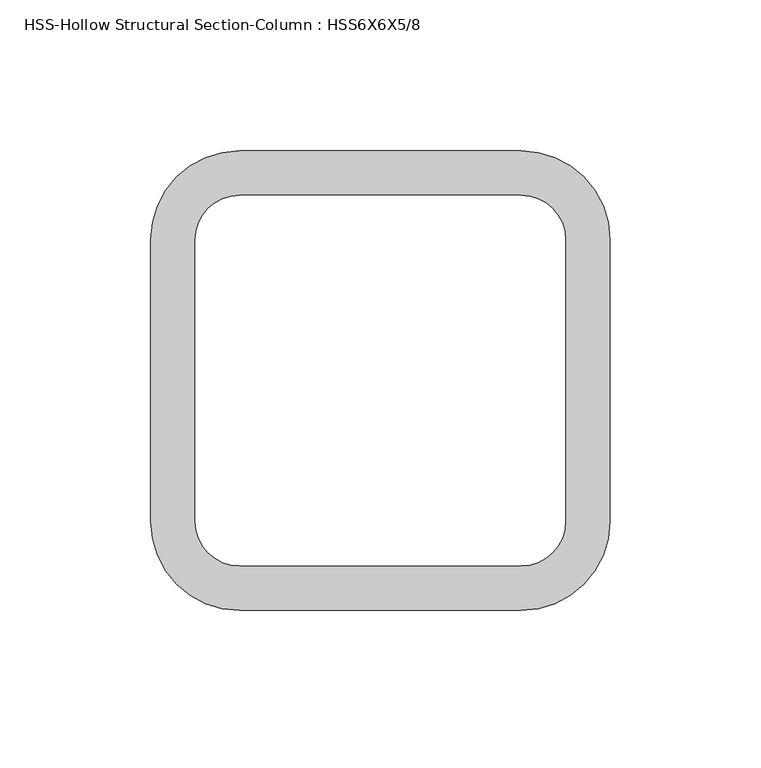
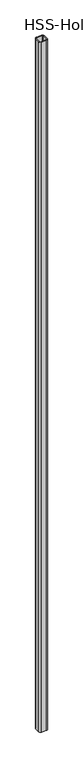
"""IFC4 building model written with IfcOpenShell, lengths in millimetres: column geometry, HSS-Hollow Structural Section-Column : HSS6X6X5/8."""

from ifc_helpers import new_model, si_unit, point, frame, frame_2d, origin, place, context, project, spatial, polyline, circle_curve, trimmed, segment, composite_curve, outline, extrude, source, transform, mapped, element, save


def hss_hollow_structural_section_column_hss6x6x5_8_b8f4d47c(model_context):
    return source(origin(), model_context, "Body", "SweptSolid", [
        extrude(outline(composite_curve([segment(trimmed(circle_curve(frame_2d((46.6852, 46.6852)), 29.5148), [point((46.6852, 76.2))], [point((76.2, 46.6852))], False, "CARTESIAN"), True, "CONTINUOUS"), segment(polyline([(76.2, 46.6852), (76.2, -46.6852)]), True, "CONTINUOUS"), segment(trimmed(circle_curve(frame_2d((46.6852, -46.6852)), 29.5148), [point((76.2, -46.6852))], [point((46.6852, -76.2))], False, "CARTESIAN"), True, "CONTINUOUS"), segment(polyline([(46.6852, -76.2), (-46.6852, -76.2)]), True, "CONTINUOUS"), segment(trimmed(circle_curve(frame_2d((-46.6852, -46.6852)), 29.5148), [point((-46.6852, -76.2))], [point((-76.2, -46.6852))], False, "CARTESIAN"), True, "CONTINUOUS"), segment(polyline([(-76.2, -46.6852), (-76.2, 46.6852)]), True, "CONTINUOUS"), segment(trimmed(circle_curve(frame_2d((-46.6852, 46.6852)), 29.5148), [point((-76.2, 46.6852))], [point((-46.6852, 76.2))], False, "CARTESIAN"), True, "CONTINUOUS"), segment(polyline([(-46.6852, 76.2), (46.6852, 76.2)]), True, "CONTINUOUS")], self_intersect=False), holes=[composite_curve([segment(polyline([(46.6852, 61.4426), (-46.6852, 61.4426)]), True, "CONTINUOUS"), segment(trimmed(circle_curve(frame_2d((-46.6852, 46.6852)), 14.7574), [point((-46.6852, 61.4426))], [point((-61.4426, 46.6852))], True, "CARTESIAN"), True, "CONTINUOUS"), segment(polyline([(-61.4426, 46.6852), (-61.4426, -46.6852)]), True, "CONTINUOUS"), segment(trimmed(circle_curve(frame_2d((-46.6852, -46.6852)), 14.7574), [point((-61.4426, -46.6852))], [point((-46.6852, -61.4426))], True, "CARTESIAN"), True, "CONTINUOUS"), segment(polyline([(-46.6852, -61.4426), (46.6852, -61.4426)]), True, "CONTINUOUS"), segment(trimmed(circle_curve(frame_2d((46.6852, -46.6852)), 14.7574), [point((46.6852, -61.4426))], [point((61.4426, -46.6852))], True, "CARTESIAN"), True, "CONTINUOUS"), segment(polyline([(61.4426, -46.6852), (61.4426, 46.6852)]), True, "CONTINUOUS"), segment(trimmed(circle_curve(frame_2d((46.6852, 46.6852)), 14.7574), [point((61.4426, 46.6852))], [point((46.6852, 61.4426))], True, "CARTESIAN"), True, "CONTINUOUS")], self_intersect=False)]), frame((0.0, 0.0, -609.6), z_axis=(0.0, 0.0, 1.0), x_axis=(1.0, 0.0, 0.0)), (0.0, 0.0, 1.0), 12877.8),
    ])


if __name__ == "__main__":
    model = new_model("IFC4")
    model_context = context("Model", 3, world=origin())
    ifc_project = project(units=[si_unit("LENGTHUNIT", "METRE", prefix="MILLI")], contexts=[model_context])
    site = spatial("IfcSite", under=ifc_project)
    building = spatial("IfcBuilding", under=site)
    placement = place(None, origin())
    hss_hollow_structural_section_column_hss6x6x5_8_shape = hss_hollow_structural_section_column_hss6x6x5_8_b8f4d47c(model_context)
    element("IfcColumn", 1, ObjectType="HSS-Hollow Structural Section-Column : HSS6X6X5/8", at=placement, inside=building, context=model_context, shape_type="MappedRepresentation", body=[
        mapped(hss_hollow_structural_section_column_hss6x6x5_8_shape, transform((0.0, 0.0, 0.0), x_axis=(1.0, 0.0, 0.0), y_axis=(0.0, 1.0, 0.0), z_axis=(0.0, 0.0, 1.0))),
    ])
    save(model, "model.ifc")

# Revit data of these elements
# Type "HSS-Hollow Structural Section-Column : HSS6X6X5/8"
#   Assembly Code = "B10"
#   Shape = "Square"
#   W = 42.1
#   Ht = 0' - 6"
#   b = 0' - 6"
#   kr = 0' - 1.162"
#   t = 0' - 0.581"
#   A = 0.08125 SF
#   Structural Material [instance default] = Steel ASTM A500, Grade B, Rectangular and Square
# Element 1 (IfcColumn, "HSS-Hollow Structural Section-Column : HSS6X6X5/8")
#   Materials on its faces: "Steel ASTM A500, Grade B, Rectangular and Square"
# Materials
#   "Steel ASTM A500, Grade B, Rectangular and Square": class "Metal", colour RGB 199 199 199, transparency 0, Description = "Carbon steel", Cost = 0
